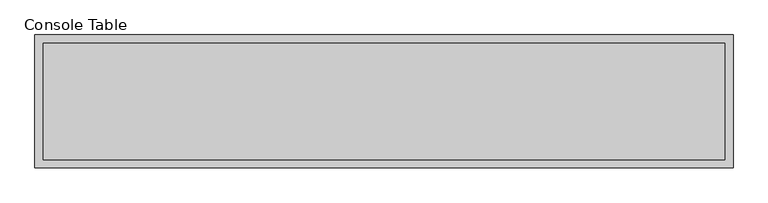
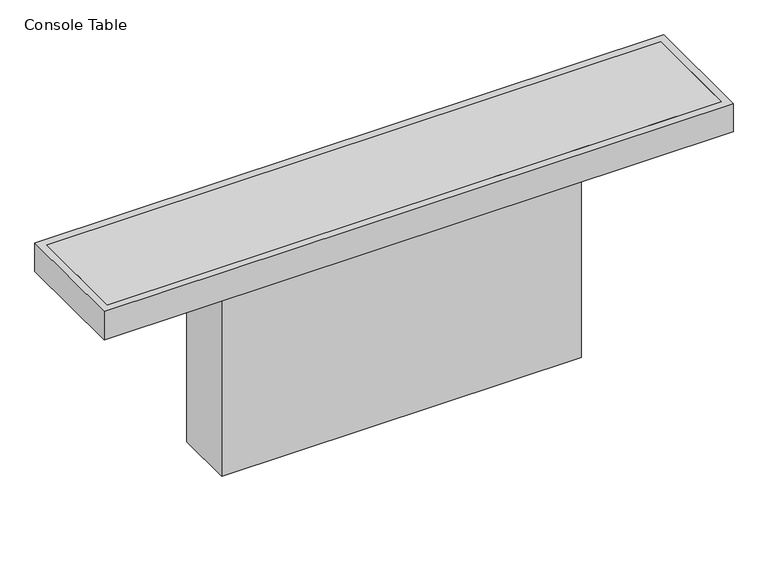
"""IFC4 building model written with IfcOpenShell, lengths in millimetres: furniture geometry, Console Table."""

import ifcopenshell
import ifcopenshell.guid

model = None  # the IFC model being written
_history = None  # IfcOwnerHistory: only IFC2X3 demands one
_inside = {}  # id of a spatial element -> (the spatial element, [elements in it])
_under = {}  # id of a project, library or spatial element -> (it, [spatial elements below it])
_declared = {}  # id of a project -> (the project, [libraries it declares])
_typed = {}  # id of a type object -> (the type object, [elements of that type])
_made_of = {}  # id of a material, layer set ... -> (it, [elements and type objects made of it])


def new_model(schema):
    """Start an empty IFC model of exactly this schema.

    Asked for "IFC4X3", IfcOpenShell would pick the latest addendum, in which some entities
    have other attributes; the version numbers below select the first issue.
    IFC2X3 requires an IfcOwnerHistory on every rooted entity: one is made here for all.
    """
    global model, _history
    if schema == "IFC4X3":
        model = ifcopenshell.file(schema_version=(4, 3, 0, 0))
    else:
        model = ifcopenshell.file(schema=schema)
    _inside.clear()
    _under.clear()
    _declared.clear()
    _typed.clear()
    _made_of.clear()
    _history = None
    if model.schema == "IFC2X3":
        org = make("IfcOrganization", Name="unknown")
        user = make(
            "IfcPersonAndOrganization",
            ThePerson=make("IfcPerson", FamilyName="unknown"),
            TheOrganization=org,
        )
        app = make(
            "IfcApplication",
            ApplicationDeveloper=org,
            Version="unknown",
            ApplicationFullName="unknown",
            ApplicationIdentifier="unknown",
        )
        _history = make(
            "IfcOwnerHistory",
            OwningUser=user,
            OwningApplication=app,
            ChangeAction="ADDED",
            CreationDate=0,
        )
    return model


def make(cls, **values):
    """One entity of the class cls with the attributes given. An attribute that is None is left unset."""
    return model.create_entity(
        cls, **{name: value for name, value in values.items() if value is not None}
    )


def rooted(cls, **values):
    """An entity with a GlobalId (a new one), such as an element, a storey or a relation."""
    return make(cls, GlobalId=ifcopenshell.guid.new(), OwnerHistory=_history, **values)


def si_unit(unit_type, name, prefix=None):
    """IfcSIUnit, for example si_unit("LENGTHUNIT", "METRE", prefix="MILLI")."""
    return make("IfcSIUnit", UnitType=unit_type, Prefix=prefix, Name=name)


def assignment(units):
    """IfcUnitAssignment: the units of a project."""
    return None if units is None else make("IfcUnitAssignment", Units=units)


def point(xyz):
    """IfcCartesianPoint."""
    return None if xyz is None else make("IfcCartesianPoint", Coordinates=xyz)


def direction(xyz):
    """IfcDirection."""
    return None if xyz is None else make("IfcDirection", DirectionRatios=xyz)


def frame(location, z_axis=None, x_axis=None):
    """IfcAxis2Placement3D, a coordinate frame: its origin and axes. An axis left out is left unset."""
    return make(
        "IfcAxis2Placement3D",
        Location=point(location),
        Axis=direction(z_axis),
        RefDirection=direction(x_axis),
    )


def origin():
    """The frame at (0, 0, 0) with its axes left unset."""
    return frame((0.0, 0.0, 0.0))


def origin_with_axes():
    """The frame at (0, 0, 0) with the z axis (0, 0, 1) and the x axis (1, 0, 0) written out."""
    return frame((0.0, 0.0, 0.0), z_axis=(0.0, 0.0, 1.0), x_axis=(1.0, 0.0, 0.0))


def place(relative_to, where):
    """IfcLocalPlacement: puts the frame where relative to a parent placement (None: the world)."""
    return make(
        "IfcLocalPlacement", PlacementRelTo=relative_to, RelativePlacement=where
    )


def context(
    kind, dimensions, precision=None, world=None, true_north=None, identifier=None
):
    """IfcGeometricRepresentationContext, for example the 3D "Model" context."""
    return make(
        "IfcGeometricRepresentationContext",
        ContextIdentifier=identifier,
        ContextType=kind,
        CoordinateSpaceDimension=dimensions,
        Precision=precision,
        WorldCoordinateSystem=world,
        TrueNorth=true_north,
    )


def project(units=None, contexts=None):
    """IfcProject with its units and contexts."""
    return rooted(
        "IfcProject",
        Name="project",
        RepresentationContexts=contexts,
        UnitsInContext=assignment(units),
    )


def spatial(cls, under=None, at=None, **own):
    """A site, building, storey or space (cls), placed at a placement, below another one or the project."""
    s = rooted(cls, ObjectPlacement=at, **own)
    if under is not None:
        _under.setdefault(under.id(), (under, []))[1].append(s)
    return s


def polyline(points):
    """IfcPolyline through the points."""
    return make("IfcPolyline", Points=[point(p) for p in points])


def outline(outer, holes=None, kind="AREA"):
    """IfcArbitraryClosedProfileDef: a profile drawn as a closed curve; with holes, ...WithVoids."""
    if holes is None:
        return make("IfcArbitraryClosedProfileDef", ProfileType=kind, OuterCurve=outer)
    return make(
        "IfcArbitraryProfileDefWithVoids",
        ProfileType=kind,
        OuterCurve=outer,
        InnerCurves=holes,
    )


def extrude(swept, where, along, depth):
    """IfcExtrudedAreaSolid: the profile swept, set in the frame where, extruded along a direction by depth."""
    return make(
        "IfcExtrudedAreaSolid",
        SweptArea=swept,
        Position=where,
        ExtrudedDirection=direction(along),
        Depth=depth,
    )


def shape(context_of_items, identifier, shape_type, items):
    """IfcShapeRepresentation: the items that make up one representation, for example the "Body"."""
    return make(
        "IfcShapeRepresentation",
        ContextOfItems=context_of_items,
        RepresentationIdentifier=identifier,
        RepresentationType=shape_type,
        Items=items,
    )


def source(mapping_origin, context_of_items, identifier, shape_type, items):
    """IfcRepresentationMap: a shape defined once, which mapped items show again and again."""
    return make(
        "IfcRepresentationMap",
        MappingOrigin=mapping_origin,
        MappedRepresentation=shape(context_of_items, identifier, shape_type, items),
    )


def transform(
    local_origin,
    x_axis=None,
    y_axis=None,
    z_axis=None,
    scale=None,
    scale2=None,
    scale3=None,
    uniform=True,
):
    """IfcCartesianTransformationOperator3D, or its non-uniform kind. x_axis, y_axis, z_axis: its Axis1, 2, 3."""
    if uniform:
        return make(
            "IfcCartesianTransformationOperator3D",
            Axis1=direction(x_axis),
            Axis2=direction(y_axis),
            LocalOrigin=point(local_origin),
            Scale=scale,
            Axis3=direction(z_axis),
        )
    return make(
        "IfcCartesianTransformationOperator3DnonUniform",
        Axis1=direction(x_axis),
        Axis2=direction(y_axis),
        LocalOrigin=point(local_origin),
        Scale=scale,
        Axis3=direction(z_axis),
        Scale2=scale2,
        Scale3=scale3,
    )


def mapped(mapping_source, mapping_target):
    """IfcMappedItem: shows the shape of a source again, moved by a transform."""
    return make(
        "IfcMappedItem", MappingSource=mapping_source, MappingTarget=mapping_target
    )


def made_of(thing, what):
    """Note that an element or type object is made of a material, layer set ...; save() writes the relation."""
    if what is not None:
        _made_of.setdefault(what.id(), (what, []))[1].append(thing)
    return thing


def element(
    cls,
    number,
    at=None,
    inside=None,
    cuts=None,
    type_object=None,
    material=None,
    context=None,
    identifier="Body",
    shape_type=None,
    held_by="IfcProductDefinitionShape",
    body=None,
    shapes=None,
    **own,
):
    """One element of the class cls, such as IfcWall. Its Tag is "e" and its number.

    at: its placement. inside: the storey or other place that contains it. cuts: it is an
    opening in that element (IfcRelVoidsElement). A single representation is given by context,
    identifier, shape_type and body (its items); several are given by shapes. held_by: the class
    of the entity that holds the representations. save() writes the other relations.
    """
    e = rooted(cls, Tag="e%d" % number, ObjectPlacement=at, **own)
    if body is not None:
        shapes = [shape(context, identifier, shape_type, body)]
    if shapes is not None:
        e.Representation = make(held_by, Representations=shapes)
    if inside is not None:
        _inside.setdefault(inside.id(), (inside, []))[1].append(e)
    if cuts is not None:
        rooted(
            "IfcRelVoidsElement", RelatingBuildingElement=cuts, RelatedOpeningElement=e
        )
    if type_object is not None:
        _typed.setdefault(type_object.id(), (type_object, []))[1].append(e)
    return made_of(e, material)


def aggregate(whole, parts):
    """IfcRelAggregates: a whole, such as a stair, and the parts it consists of."""
    return rooted("IfcRelAggregates", RelatingObject=whole, RelatedObjects=parts)


def save(model, path):
    """Write the relations noted so far, then the file.

    IfcRelAggregates (storeys below a building ...), IfcRelContainedInSpatialStructure (elements
    in a storey), IfcRelDefinesByType, IfcRelAssociatesMaterial and IfcRelDeclares: one each for
    every whole, place, type object, material and project.
    """
    for whole, parts in _under.values():
        aggregate(whole, parts)
    for where, things in _inside.values():
        rooted(
            "IfcRelContainedInSpatialStructure",
            RelatedElements=things,
            RelatingStructure=where,
        )
    for kind, things in _typed.values():
        rooted("IfcRelDefinesByType", RelatedObjects=things, RelatingType=kind)
    for what, things in _made_of.values():
        rooted("IfcRelAssociatesMaterial", RelatedObjects=things, RelatingMaterial=what)
    for by, libraries in _declared.values():
        rooted("IfcRelDeclares", RelatingContext=by, RelatedDefinitions=libraries)
    model.write(path)


def console_table_7339a461(model_context):
    return source(origin(), model_context, "Body", "SweptSolid", [
        extrude(outline(polyline([(609.6, 101.6), (609.6, -101.6), (-609.6, -101.6), (-609.6, 101.6), (609.6, 101.6)])), origin_with_axes(), (0.0, 0.0, 1.0), 787.4),
        extrude(outline(polyline([(-1041.4, -177.8), (-1041.4, 177.8), (1041.4, 177.8), (1041.4, -177.8), (-1041.4, -177.8)])), frame((0.0, 0.0, 787.4), z_axis=(0.0, 0.0, 1.0), x_axis=(1.0, 0.0, 0.0)), (0.0, 0.0, 1.0), 25.4),
        extrude(outline(polyline([(1066.8, 203.2), (1066.8, -203.2), (-1066.8, -203.2), (-1066.8, 203.2), (1066.8, 203.2)]), holes=[polyline([(1041.4, 177.8), (-1041.4, 177.8), (-1041.4, -177.8), (1041.4, -177.8), (1041.4, 177.8)])]), frame((0.0, 0.0, 711.2), z_axis=(0.0, 0.0, 1.0), x_axis=(1.0, 0.0, 0.0)), (0.0, 0.0, 1.0), 101.6),
    ])


if __name__ == "__main__":
    model = new_model("IFC4")
    model_context = context("Model", 3, world=origin())
    ifc_project = project(units=[si_unit("LENGTHUNIT", "METRE", prefix="MILLI")], contexts=[model_context])
    site = spatial("IfcSite", under=ifc_project)
    building = spatial("IfcBuilding", under=site)
    placement = place(None, origin())
    console_table_shape = console_table_7339a461(model_context)
    element("IfcFurniture", 1, ObjectType="Console Table : 84\" L x 16\" W x 32\" H", at=placement, inside=building, context=model_context, shape_type="MappedRepresentation", body=[
        mapped(console_table_shape, transform((0.0, 0.0, 0.0), x_axis=(1.0, 0.0, 0.0), y_axis=(0.0, 1.0, 0.0), z_axis=(0.0, 0.0, 1.0))),
    ])
    save(model, "model.ifc")

# Revit data of these elements
# Type "Console Table : 84\" L x 16\" W x 32\" H"
#   Table Width = 406.40 mm
#   Table Length = 2133.60 mm
#   Table Height = 812.80 mm
#   Pedestal Width = 203.20 mm
#   Pedestal Length = 1219.20 mm
#   Frame Thickness = 25.40 mm
#   Frame Height = 101.60 mm
#   Table Surface [instance default] = none
#   Table Frame [instance default] = none
#   Pedestal [instance default] = none
#   Assembly Code = ""
